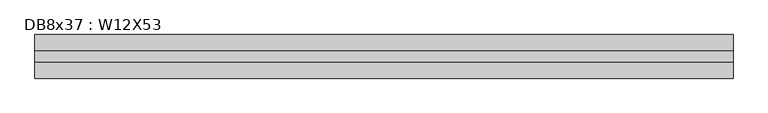
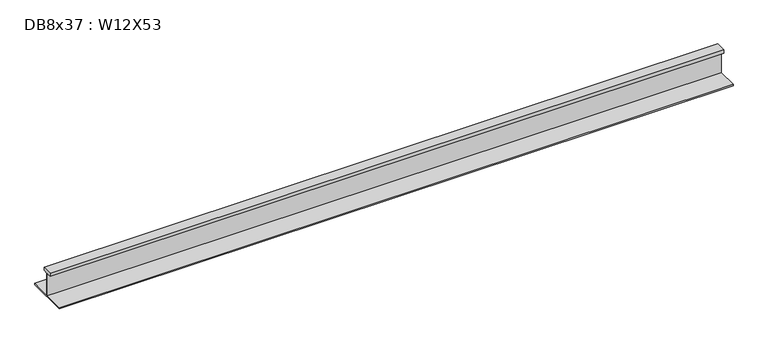
"""IFC4 building model written with IfcOpenShell, lengths in millimetres: beam geometry, DB8x37 : W12X53."""

from ifc_helpers import new_model, si_unit, frame, origin, place, context, project, spatial, polyline, outline, extrude, source, transform, mapped, element, save


def db8x37_w12x53_d062fcd9(model_context):
    return source(origin(), model_context, "Body", "SweptSolid", [
        extrude(outline(polyline([(38.1, 145.415), (38.1, 120.015), (2.921, 120.015), (2.921, -48.4505), (152.4, -48.4505), (152.4, -58.1025), (-152.4, -58.1025), (-152.4, -48.4505), (-2.921, -48.4505), (-2.921, 120.015), (-38.1, 120.015), (-38.1, 145.415), (38.1, 145.415)])), frame((-2451.608, 0.0, 0.0), z_axis=(1.0, 0.0, 0.0), x_axis=(0.0, 1.0, 0.0)), (0.0, 0.0, 1.0), 4880.737),
    ])


if __name__ == "__main__":
    model = new_model("IFC4")
    model_context = context("Model", 3, world=origin())
    ifc_project = project(units=[si_unit("LENGTHUNIT", "METRE", prefix="MILLI")], contexts=[model_context])
    site = spatial("IfcSite", under=ifc_project)
    building = spatial("IfcBuilding", under=site)
    placement = place(None, origin())
    db8x37_w12x53_shape = db8x37_w12x53_d062fcd9(model_context)
    element("IfcBeam", 1, ObjectType="DB8x37 : W12X53", at=placement, inside=building, context=model_context, shape_type="MappedRepresentation", body=[
        mapped(db8x37_w12x53_shape, transform((0.0, 0.0, 0.0), x_axis=(1.0, 0.0, 0.0), y_axis=(0.0, 1.0, 0.0), z_axis=(0.0, 0.0, 1.0))),
    ])
    save(model, "model.ifc")

# Revit data of these elements
# Type "DB8x37 : W12X53"
#   Assembly Code = "B10"
#   W = 53
#   Length [instance default] = 5' - 0"
#   bf = 0' - 10"
#   d = 1' - 0.1"
#   k = 0' - 1 3/8"
#   k2 = 0' - 0.8"
#   tf = 0' - 0.575"
#   tw = 0' - 0.345"
#   A = 0.108333 SF
#   Structural Material [instance default] = Steel ASTM A992
# Element 1 (IfcBeam, "DB8x37 : W12X53")
#   Materials on its faces: "Steel ASTM A992"
# Materials
#   "Steel ASTM A992": class "Metal", colour RGB 199 199 199, transparency 0, Description = "Structural steel 50ksi", Cost = 0
